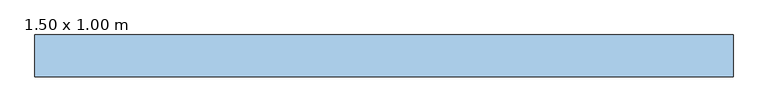
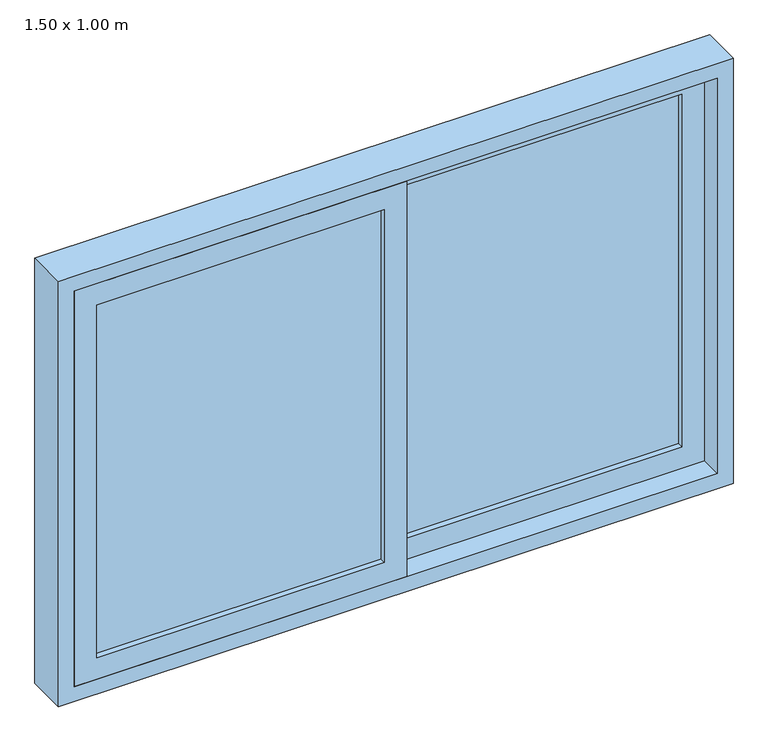
"""IFC4 building model written with IfcOpenShell, lengths in millimetres: window geometry, Janela de correr vidro - 2 Folhas : 1.50 x 1.00 m."""

import ifcopenshell
import ifcopenshell.guid

model = None  # the IFC model being written
_history = None  # IfcOwnerHistory: only IFC2X3 demands one
_inside = {}  # id of a spatial element -> (the spatial element, [elements in it])
_under = {}  # id of a project, library or spatial element -> (it, [spatial elements below it])
_declared = {}  # id of a project -> (the project, [libraries it declares])
_typed = {}  # id of a type object -> (the type object, [elements of that type])
_made_of = {}  # id of a material, layer set ... -> (it, [elements and type objects made of it])


def new_model(schema):
    """Start an empty IFC model of exactly this schema.

    Asked for "IFC4X3", IfcOpenShell would pick the latest addendum, in which some entities
    have other attributes; the version numbers below select the first issue.
    IFC2X3 requires an IfcOwnerHistory on every rooted entity: one is made here for all.
    """
    global model, _history
    if schema == "IFC4X3":
        model = ifcopenshell.file(schema_version=(4, 3, 0, 0))
    else:
        model = ifcopenshell.file(schema=schema)
    _inside.clear()
    _under.clear()
    _declared.clear()
    _typed.clear()
    _made_of.clear()
    _history = None
    if model.schema == "IFC2X3":
        org = make("IfcOrganization", Name="unknown")
        user = make(
            "IfcPersonAndOrganization",
            ThePerson=make("IfcPerson", FamilyName="unknown"),
            TheOrganization=org,
        )
        app = make(
            "IfcApplication",
            ApplicationDeveloper=org,
            Version="unknown",
            ApplicationFullName="unknown",
            ApplicationIdentifier="unknown",
        )
        _history = make(
            "IfcOwnerHistory",
            OwningUser=user,
            OwningApplication=app,
            ChangeAction="ADDED",
            CreationDate=0,
        )
    return model


def make(cls, **values):
    """One entity of the class cls with the attributes given. An attribute that is None is left unset."""
    return model.create_entity(
        cls, **{name: value for name, value in values.items() if value is not None}
    )


def rooted(cls, **values):
    """An entity with a GlobalId (a new one), such as an element, a storey or a relation."""
    return make(cls, GlobalId=ifcopenshell.guid.new(), OwnerHistory=_history, **values)


def si_unit(unit_type, name, prefix=None):
    """IfcSIUnit, for example si_unit("LENGTHUNIT", "METRE", prefix="MILLI")."""
    return make("IfcSIUnit", UnitType=unit_type, Prefix=prefix, Name=name)


def assignment(units):
    """IfcUnitAssignment: the units of a project."""
    return None if units is None else make("IfcUnitAssignment", Units=units)


def point(xyz):
    """IfcCartesianPoint."""
    return None if xyz is None else make("IfcCartesianPoint", Coordinates=xyz)


def direction(xyz):
    """IfcDirection."""
    return None if xyz is None else make("IfcDirection", DirectionRatios=xyz)


def frame(location, z_axis=None, x_axis=None):
    """IfcAxis2Placement3D, a coordinate frame: its origin and axes. An axis left out is left unset."""
    return make(
        "IfcAxis2Placement3D",
        Location=point(location),
        Axis=direction(z_axis),
        RefDirection=direction(x_axis),
    )


def origin():
    """The frame at (0, 0, 0) with its axes left unset."""
    return frame((0.0, 0.0, 0.0))


def place(relative_to, where):
    """IfcLocalPlacement: puts the frame where relative to a parent placement (None: the world)."""
    return make(
        "IfcLocalPlacement", PlacementRelTo=relative_to, RelativePlacement=where
    )


def context(
    kind, dimensions, precision=None, world=None, true_north=None, identifier=None
):
    """IfcGeometricRepresentationContext, for example the 3D "Model" context."""
    return make(
        "IfcGeometricRepresentationContext",
        ContextIdentifier=identifier,
        ContextType=kind,
        CoordinateSpaceDimension=dimensions,
        Precision=precision,
        WorldCoordinateSystem=world,
        TrueNorth=true_north,
    )


def project(units=None, contexts=None):
    """IfcProject with its units and contexts."""
    return rooted(
        "IfcProject",
        Name="project",
        RepresentationContexts=contexts,
        UnitsInContext=assignment(units),
    )


def spatial(cls, under=None, at=None, **own):
    """A site, building, storey or space (cls), placed at a placement, below another one or the project."""
    s = rooted(cls, ObjectPlacement=at, **own)
    if under is not None:
        _under.setdefault(under.id(), (under, []))[1].append(s)
    return s


def polyline(points):
    """IfcPolyline through the points."""
    return make("IfcPolyline", Points=[point(p) for p in points])


def outline(outer, holes=None, kind="AREA"):
    """IfcArbitraryClosedProfileDef: a profile drawn as a closed curve; with holes, ...WithVoids."""
    if holes is None:
        return make("IfcArbitraryClosedProfileDef", ProfileType=kind, OuterCurve=outer)
    return make(
        "IfcArbitraryProfileDefWithVoids",
        ProfileType=kind,
        OuterCurve=outer,
        InnerCurves=holes,
    )


def extrude(swept, where, along, depth):
    """IfcExtrudedAreaSolid: the profile swept, set in the frame where, extruded along a direction by depth."""
    return make(
        "IfcExtrudedAreaSolid",
        SweptArea=swept,
        Position=where,
        ExtrudedDirection=direction(along),
        Depth=depth,
    )


def shape(context_of_items, identifier, shape_type, items):
    """IfcShapeRepresentation: the items that make up one representation, for example the "Body"."""
    return make(
        "IfcShapeRepresentation",
        ContextOfItems=context_of_items,
        RepresentationIdentifier=identifier,
        RepresentationType=shape_type,
        Items=items,
    )


def source(mapping_origin, context_of_items, identifier, shape_type, items):
    """IfcRepresentationMap: a shape defined once, which mapped items show again and again."""
    return make(
        "IfcRepresentationMap",
        MappingOrigin=mapping_origin,
        MappedRepresentation=shape(context_of_items, identifier, shape_type, items),
    )


def transform(
    local_origin,
    x_axis=None,
    y_axis=None,
    z_axis=None,
    scale=None,
    scale2=None,
    scale3=None,
    uniform=True,
):
    """IfcCartesianTransformationOperator3D, or its non-uniform kind. x_axis, y_axis, z_axis: its Axis1, 2, 3."""
    if uniform:
        return make(
            "IfcCartesianTransformationOperator3D",
            Axis1=direction(x_axis),
            Axis2=direction(y_axis),
            LocalOrigin=point(local_origin),
            Scale=scale,
            Axis3=direction(z_axis),
        )
    return make(
        "IfcCartesianTransformationOperator3DnonUniform",
        Axis1=direction(x_axis),
        Axis2=direction(y_axis),
        LocalOrigin=point(local_origin),
        Scale=scale,
        Axis3=direction(z_axis),
        Scale2=scale2,
        Scale3=scale3,
    )


def mapped(mapping_source, mapping_target):
    """IfcMappedItem: shows the shape of a source again, moved by a transform."""
    return make(
        "IfcMappedItem", MappingSource=mapping_source, MappingTarget=mapping_target
    )


def made_of(thing, what):
    """Note that an element or type object is made of a material, layer set ...; save() writes the relation."""
    if what is not None:
        _made_of.setdefault(what.id(), (what, []))[1].append(thing)
    return thing


def element(
    cls,
    number,
    at=None,
    inside=None,
    cuts=None,
    type_object=None,
    material=None,
    context=None,
    identifier="Body",
    shape_type=None,
    held_by="IfcProductDefinitionShape",
    body=None,
    shapes=None,
    **own,
):
    """One element of the class cls, such as IfcWall. Its Tag is "e" and its number.

    at: its placement. inside: the storey or other place that contains it. cuts: it is an
    opening in that element (IfcRelVoidsElement). A single representation is given by context,
    identifier, shape_type and body (its items); several are given by shapes. held_by: the class
    of the entity that holds the representations. save() writes the other relations.
    """
    e = rooted(cls, Tag="e%d" % number, ObjectPlacement=at, **own)
    if body is not None:
        shapes = [shape(context, identifier, shape_type, body)]
    if shapes is not None:
        e.Representation = make(held_by, Representations=shapes)
    if inside is not None:
        _inside.setdefault(inside.id(), (inside, []))[1].append(e)
    if cuts is not None:
        rooted(
            "IfcRelVoidsElement", RelatingBuildingElement=cuts, RelatedOpeningElement=e
        )
    if type_object is not None:
        _typed.setdefault(type_object.id(), (type_object, []))[1].append(e)
    return made_of(e, material)


def aggregate(whole, parts):
    """IfcRelAggregates: a whole, such as a stair, and the parts it consists of."""
    return rooted("IfcRelAggregates", RelatingObject=whole, RelatedObjects=parts)


def save(model, path):
    """Write the relations noted so far, then the file.

    IfcRelAggregates (storeys below a building ...), IfcRelContainedInSpatialStructure (elements
    in a storey), IfcRelDefinesByType, IfcRelAssociatesMaterial and IfcRelDeclares: one each for
    every whole, place, type object, material and project.
    """
    for whole, parts in _under.values():
        aggregate(whole, parts)
    for where, things in _inside.values():
        rooted(
            "IfcRelContainedInSpatialStructure",
            RelatedElements=things,
            RelatingStructure=where,
        )
    for kind, things in _typed.values():
        rooted("IfcRelDefinesByType", RelatedObjects=things, RelatingType=kind)
    for what, things in _made_of.values():
        rooted("IfcRelAssociatesMaterial", RelatedObjects=things, RelatingMaterial=what)
    for by, libraries in _declared.values():
        rooted("IfcRelDeclares", RelatingContext=by, RelatedDefinitions=libraries)
    model.write(path)


def window_1_50_x_1_00_m_3664bad9(model_context):
    return source(origin(), model_context, "Body", "SweptSolid", [
        extrude(outline(polyline([(935.0, -25.0), (935.0, 715.0), (1865.0, 715.0), (1865.0, -25.0), (935.0, -25.0)]), holes=[polyline([(1815.0, 25.0), (1815.0, 665.0), (985.0, 665.0), (985.0, 25.0), (1815.0, 25.0)])]), frame((0.0, -35.0, 0.0), z_axis=(0.0, 1.0, 0.0), x_axis=(0.0, 0.0, 1.0)), (0.0, 0.0, 1.0), 40.0),
        extrude(outline(polyline([(1865.0, 25.0), (1865.0, -715.0), (935.0, -715.0), (935.0, 25.0), (1865.0, 25.0)]), holes=[polyline([(985.0, -25.0), (985.0, -665.0), (1815.0, -665.0), (1815.0, -25.0), (985.0, -25.0)])]), frame((0.0, -85.0, 0.0), z_axis=(0.0, 1.0, 0.0), x_axis=(0.0, 0.0, 1.0)), (0.0, 0.0, 1.0), 40.0),
        extrude(outline(polyline([(1900.0, 750.0), (1900.0, -750.0), (900.0, -750.0), (900.0, 750.0), (1900.0, 750.0)]), holes=[polyline([(935.0, 715.0), (935.0, -715.0), (1865.0, -715.0), (1865.0, 715.0), (935.0, 715.0)])]), frame((0.0, -85.0, 0.0), z_axis=(0.0, 1.0, 0.0), x_axis=(0.0, 0.0, 1.0)), (0.0, 0.0, 1.0), 90.0),
        extrude(outline(polyline([(25.0, -8.0), (665.0, -8.0), (665.0, -22.0), (25.0, -22.0), (25.0, -8.0)])), frame((0.0, 0.0, 985.0), z_axis=(0.0, 0.0, 1.0), x_axis=(1.0, 0.0, 0.0)), (0.0, 0.0, 1.0), 830.0),
        extrude(outline(polyline([(-665.0, -58.0), (-25.0, -58.0), (-25.0, -72.0), (-665.0, -72.0), (-665.0, -58.0)])), frame((0.0, 0.0, 985.0), z_axis=(0.0, 0.0, 1.0), x_axis=(1.0, 0.0, 0.0)), (0.0, 0.0, 1.0), 830.0),
    ])


if __name__ == "__main__":
    model = new_model("IFC4")
    model_context = context("Model", 3, world=origin())
    ifc_project = project(units=[si_unit("LENGTHUNIT", "METRE", prefix="MILLI")], contexts=[model_context])
    site = spatial("IfcSite", under=ifc_project)
    building = spatial("IfcBuilding", under=site)
    placement = place(None, origin())
    window_1_50_x_1_00_m_shape = window_1_50_x_1_00_m_3664bad9(model_context)
    element("IfcWindow", 1, ObjectType="Janela de correr vidro - 2 Folhas : 1.50 x 1.00 m", at=placement, inside=building, context=model_context, shape_type="MappedRepresentation", body=[
        mapped(window_1_50_x_1_00_m_shape, transform((0.0, 0.0, 0.0), x_axis=(1.0, 0.0, 0.0), y_axis=(0.0, 1.0, 0.0), z_axis=(0.0, 0.0, 1.0))),
    ])
    save(model, "model.ifc")

# Revit data of these elements
# Type "Janela de correr vidro - 2 Folhas : 1.50 x 1.00 m"
#   Type Mark = "J17"
#   Construction Type Id = "GSP4R"
#   Analytic Construction = "Vidraça única Pilkington 1/8 pol"
#   Visual Light Transmittance = 0.9
#   Thermal Resistance (R) = 0.271106 (m²·K)/W
#   Solar Heat Gain Coefficient = 0.78
#   Rough Width = 1.500 m
#   Rough Height = 1.000 m
#   Largura da moldura do painel = 0.050 m
#   Espessura da moldura do painel = 0.040 m
#   Height = 1.000 m
#   Heat Transfer Coefficient (U) = 3.6886 W/(m²·K)
#   Largura da estrutura = 0.035 m
#   Espessura da moldura = 0.090 m
#   Altura-padrão do peitoril = 0.900 m
#   Width = 1.500 m
#   Pingadeira = yes
#   Material da Pingadeira = Granito amarelo
#   Vidro = Vidro
#   Material da estrutura = Metal - Alumínio
#   Wall Closure = (empty or 0)
# Element 1 (IfcWindow, "Janela de correr vidro - 2 Folhas : 1.50 x 1.00 m")
#   Materials on its faces: "Metal - Alumínio", "Vidro"
# Materials
#   "Granito amarelo": class "Genérico", colour RGB 80 80 80, transparency 0, Cost = 0
#   "Vidro": class "Vidro", colour RGB 0 128 192, transparency 0.9
#   "Metal - Alumínio": class "Metal", colour RGB 247 247 247, transparency 0
